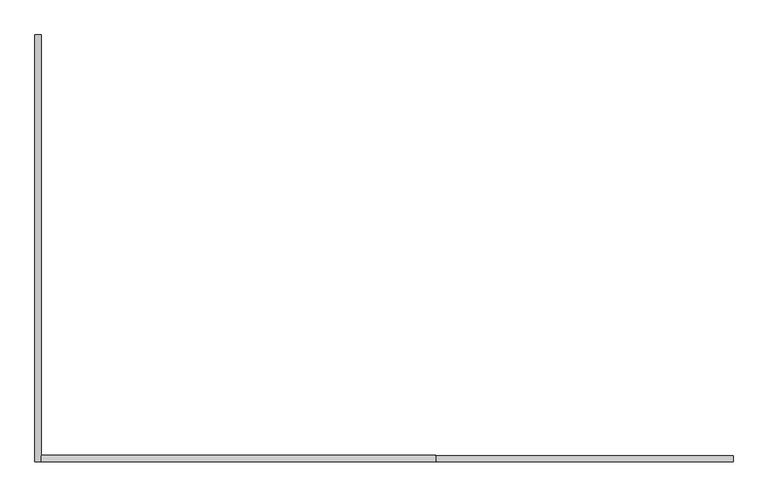
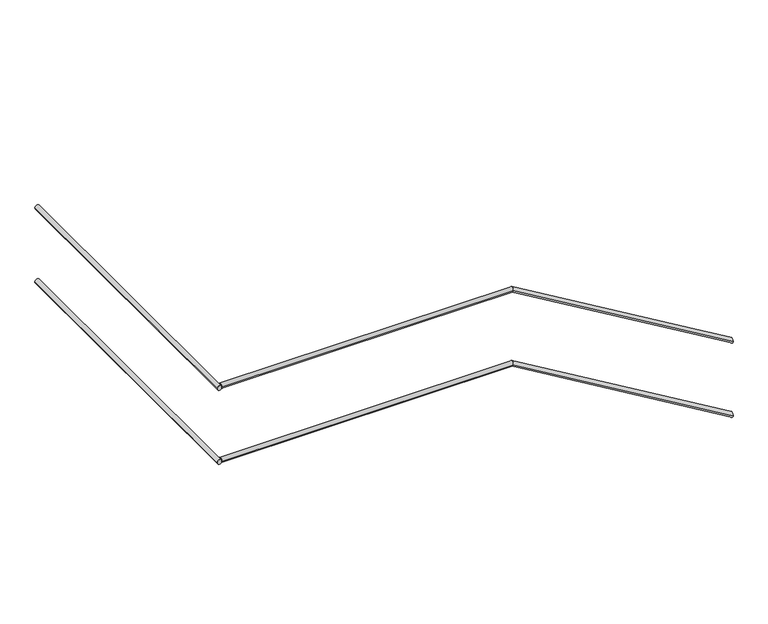
"""IFC4 building model written with IfcOpenShell, lengths in millimetres: railing geometry."""

from ifc_helpers import new_model, si_unit, frame, origin, place, context, project, spatial, circle_curve, ellipse_curve, source, transform, mapped, element, save
from ifc_brep_helpers import plane_surface, cylinder_surface, advanced_brep


def railing_fa6f35d4(model_context):
    return source(origin(), model_context, "Body", "AdvancedBrep", [
        advanced_brep(
        [(29704.7, -1668.0791411, 899.2104532), (29704.7, -1698.0791411, 899.2104532), (28300.5735614, -1668.0791411, 1735.0), (28300.5735614, -1698.0791411, 1735.0), (26440.1, -1668.0791411, 1735.0), (26440.1, -1698.0791411, 1735.0)],
        [
            (0, 1, ellipse_curve(frame((29704.7, -1683.0791411, 899.2104532), z_axis=(1.0, 0.0, 0.0), x_axis=(0.0, 0.0, -1.0)), 17.4562134, 15.0)),
            (1, 0, ellipse_curve(frame((29704.7, -1683.0791411, 899.2104532), z_axis=(1.0, 0.0, 0.0), x_axis=(0.0, 0.0, -1.0)), 17.4562134, 15.0)),
            (0, 2),
            (2, 3, ellipse_curve(frame((28300.5735614, -1683.0791411, 1735.0), z_axis=(0.9641817474962145, 0.0, -0.2652424509673105), x_axis=(-0.26524245096731125, 0.0, -0.9641817474962143)), 15.5572329, 15.0)),
            (3, 1),
            (3, 2, ellipse_curve(frame((28300.5735614, -1683.0791411, 1735.0), z_axis=(0.9641817474962145, 0.0, -0.2652424509673105), x_axis=(-0.26524245096731125, 0.0, -0.9641817474962143)), 15.5572329, 15.0)),
            (4, 5, circle_curve(frame((26440.1, -1683.0791411, 1735.0), z_axis=(-1.0, 0.0, 0.0), x_axis=(0.0, -1.0, 0.0)), 15.0)),
            (5, 4, circle_curve(frame((26440.1, -1683.0791411, 1735.0), z_axis=(-1.0, 0.0, 0.0), x_axis=(0.0, -1.0, 0.0)), 15.0)),
            (2, 4),
            (5, 3),
        ],
        [
            plane_surface(frame((29704.7, -1683.0791411, 916.6666667), z_axis=(1.0, 0.0, 0.0), x_axis=(0.0, -1.0, 0.0))),
            cylinder_surface(frame((29697.0277421, -1683.0791411, 903.7772734), z_axis=(0.8592928844097079, 0.0, -0.5114838597676807), x_axis=(0.0, -1.0, 0.0)), 15.0),
            plane_surface(frame((26440.1, -1683.0791411, 1750.0), z_axis=(-1.0, 0.0, 0.0), x_axis=(0.0, -1.0, 0.0))),
            cylinder_surface(frame((28304.7, -1683.0791411, 1735.0), z_axis=(1.0, 0.0, 0.0), x_axis=(0.0, -1.0, 0.0)), 15.0),
        ],
        [
            (0, [[1, 2]]),
            (1, [[-1, 3, 4, 5]]),
            (1, [[-2, -5, 6, -3]]),
            (2, [[7, 8]]),
            (3, [[-4, 9, -8, 10]]),
            (3, [[-6, -10, -7, -9]]),
        ],
    ),
        advanced_brep(
        [(29704.7, -1668.0791411, 1399.2104532), (29704.7, -1698.0791411, 1399.2104532), (28300.5735614, -1668.0791411, 2235.0), (28300.5735614, -1698.0791411, 2235.0), (26440.1, -1668.0791411, 2235.0), (26440.1, -1698.0791411, 2235.0)],
        [
            (0, 1, ellipse_curve(frame((29704.7, -1683.0791411, 1399.2104532), z_axis=(1.0, 0.0, 0.0), x_axis=(0.0, 0.0, -1.0)), 17.4562134, 15.0)),
            (1, 0, ellipse_curve(frame((29704.7, -1683.0791411, 1399.2104532), z_axis=(1.0, 0.0, 0.0), x_axis=(0.0, 0.0, -1.0)), 17.4562134, 15.0)),
            (0, 2),
            (2, 3, ellipse_curve(frame((28300.5735614, -1683.0791411, 2235.0), z_axis=(0.9641817474962145, 0.0, -0.2652424509673105), x_axis=(-0.26524245096731125, 0.0, -0.9641817474962143)), 15.5572329, 15.0)),
            (3, 1),
            (3, 2, ellipse_curve(frame((28300.5735614, -1683.0791411, 2235.0), z_axis=(0.9641817474962145, 0.0, -0.2652424509673105), x_axis=(-0.26524245096731125, 0.0, -0.9641817474962143)), 15.5572329, 15.0)),
            (4, 5, circle_curve(frame((26440.1, -1683.0791411, 2235.0), z_axis=(-1.0, 0.0, 0.0), x_axis=(0.0, -1.0, 0.0)), 15.0)),
            (5, 4, circle_curve(frame((26440.1, -1683.0791411, 2235.0), z_axis=(-1.0, 0.0, 0.0), x_axis=(0.0, -1.0, 0.0)), 15.0)),
            (2, 4),
            (5, 3),
        ],
        [
            plane_surface(frame((29704.7, -1683.0791411, 1416.6666667), z_axis=(1.0, 0.0, 0.0), x_axis=(0.0, -1.0, 0.0))),
            cylinder_surface(frame((29697.0277421, -1683.0791411, 1403.7772734), z_axis=(0.8592928844097079, 0.0, -0.5114838597676807), x_axis=(0.0, -1.0, 0.0)), 15.0),
            plane_surface(frame((26440.1, -1683.0791411, 2250.0), z_axis=(-1.0, 0.0, 0.0), x_axis=(0.0, -1.0, 0.0))),
            cylinder_surface(frame((28304.7, -1683.0791411, 2235.0), z_axis=(1.0, 0.0, 0.0), x_axis=(0.0, -1.0, 0.0)), 15.0),
        ],
        [
            (0, [[1, 2]]),
            (1, [[-1, 3, 4, 5]]),
            (1, [[-2, -5, 6, -3]]),
            (2, [[7, 8]]),
            (3, [[-4, 9, -8, 10]]),
            (3, [[-6, -10, -7, -9]]),
        ],
    ),
        advanced_brep(
        [(26440.1, -1698.0791411, 1735.0), (26410.1, -1698.0791411, 1735.0), (26440.1, 316.5208589, 1735.0), (26410.1, 316.5208589, 1735.0)],
        [
            (0, 1, circle_curve(frame((26425.1, -1698.0791411, 1735.0), z_axis=(0.0, -1.0, 0.0), x_axis=(-1.0, 0.0, 0.0)), 15.0)),
            (1, 0, circle_curve(frame((26425.1, -1698.0791411, 1735.0), z_axis=(0.0, -1.0, 0.0), x_axis=(-1.0, 0.0, 0.0)), 15.0)),
            (2, 3, circle_curve(frame((26425.1, 316.5208589, 1735.0), z_axis=(0.0, 1.0, 0.0), x_axis=(-1.0, 0.0, 0.0)), 15.0)),
            (3, 2, circle_curve(frame((26425.1, 316.5208589, 1735.0), z_axis=(0.0, 1.0, 0.0), x_axis=(-1.0, 0.0, 0.0)), 15.0)),
            (0, 2),
            (3, 1),
        ],
        [
            plane_surface(frame((26425.1, -1698.0791411, 1750.0), z_axis=(0.0, -1.0, 0.0), x_axis=(0.0, 0.0, 1.0))),
            plane_surface(frame((26425.1, 316.5208589, 1750.0), z_axis=(0.0, 1.0, 0.0), x_axis=(0.0, 0.0, 1.0))),
            cylinder_surface(frame((26425.1, -1698.0791411, 1735.0), z_axis=(0.0, -1.0, 0.0), x_axis=(-1.0, 0.0, 0.0)), 15.0),
        ],
        [
            (0, [[1, 2]]),
            (1, [[3, 4]]),
            (2, [[-1, 5, -4, 6]]),
            (2, [[-2, -6, -3, -5]]),
        ],
    ),
        advanced_brep(
        [(26440.1, -1698.0791411, 2235.0), (26410.1, -1698.0791411, 2235.0), (26440.1, 316.5208589, 2235.0), (26410.1, 316.5208589, 2235.0)],
        [
            (0, 1, circle_curve(frame((26425.1, -1698.0791411, 2235.0), z_axis=(0.0, -1.0, 0.0), x_axis=(-1.0, 0.0, 0.0)), 15.0)),
            (1, 0, circle_curve(frame((26425.1, -1698.0791411, 2235.0), z_axis=(0.0, -1.0, 0.0), x_axis=(-1.0, 0.0, 0.0)), 15.0)),
            (2, 3, circle_curve(frame((26425.1, 316.5208589, 2235.0), z_axis=(0.0, 1.0, 0.0), x_axis=(-1.0, 0.0, 0.0)), 15.0)),
            (3, 2, circle_curve(frame((26425.1, 316.5208589, 2235.0), z_axis=(0.0, 1.0, 0.0), x_axis=(-1.0, 0.0, 0.0)), 15.0)),
            (0, 2),
            (3, 1),
        ],
        [
            plane_surface(frame((26425.1, -1698.0791411, 2250.0), z_axis=(0.0, -1.0, 0.0), x_axis=(0.0, 0.0, 1.0))),
            plane_surface(frame((26425.1, 316.5208589, 2250.0), z_axis=(0.0, 1.0, 0.0), x_axis=(0.0, 0.0, 1.0))),
            cylinder_surface(frame((26425.1, -1698.0791411, 2235.0), z_axis=(0.0, -1.0, 0.0), x_axis=(-1.0, 0.0, 0.0)), 15.0),
        ],
        [
            (0, [[1, 2]]),
            (1, [[3, 4]]),
            (2, [[-1, 5, -4, 6]]),
            (2, [[-2, -6, -3, -5]]),
        ],
    ),
    ])


if __name__ == "__main__":
    model = new_model("IFC4")
    model_context = context("Model", 3, world=origin())
    ifc_project = project(units=[si_unit("LENGTHUNIT", "METRE", prefix="MILLI")], contexts=[model_context])
    site = spatial("IfcSite", under=ifc_project)
    building = spatial("IfcBuilding", under=site)
    placement = place(None, origin())
    railing_shape = railing_fa6f35d4(model_context)
    element("IfcRailing", 1, at=placement, inside=building, context=model_context, shape_type="MappedRepresentation", body=[
        mapped(railing_shape, transform((0.0, 0.0, 0.0), x_axis=(1.0, 0.0, 0.0), y_axis=(0.0, 1.0, 0.0), z_axis=(0.0, 0.0, 1.0))),
    ])
    save(model, "model.ifc")
